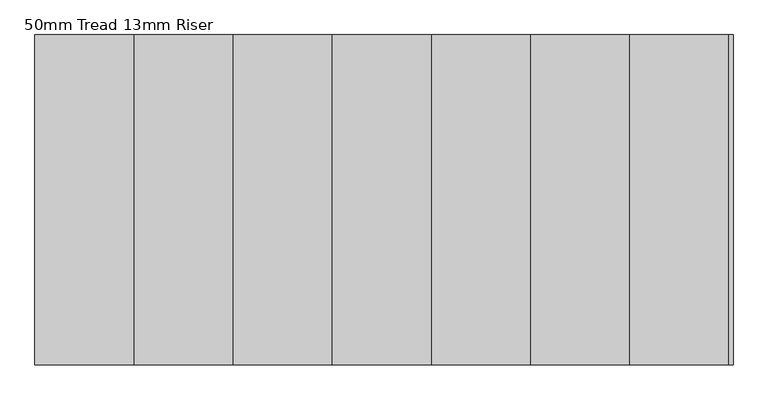
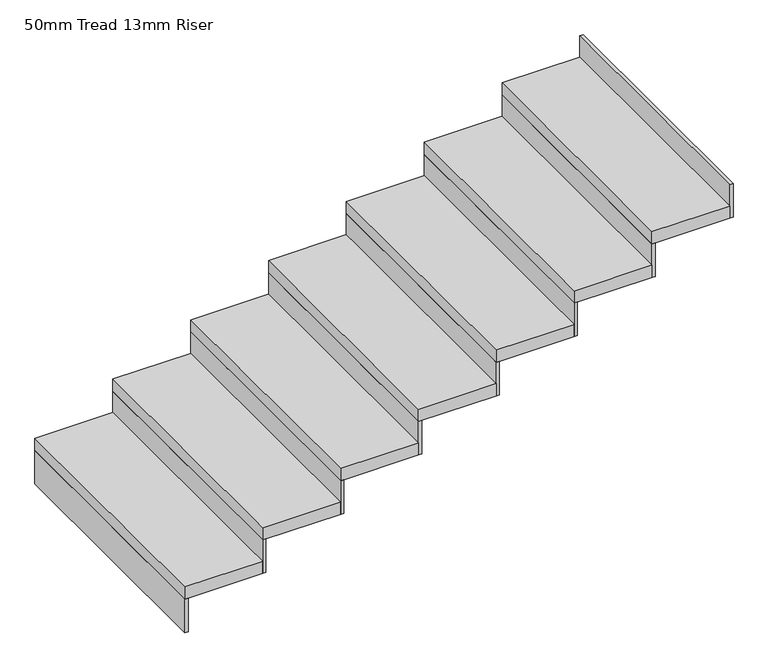
"""IFC4 building model written with IfcOpenShell, lengths in millimetres: stair flight geometry, 50mm Tread 13mm Riser."""

from ifc_helpers import new_model, si_unit, frame, origin, place, context, project, spatial, polyline, outline, extrude, source, transform, mapped, element, save


def stair_flight_50mm_tread_13mm_riser_37edc78a(model_context):
    return source(origin(), model_context, "Body", "SweptSolid", [
        extrude(outline(polyline([(-11937.8449834, -3240.1378151), (-11950.3449834, -3240.1378151), (-11950.3449834, -2240.1378151), (-11937.8449834, -2240.1378151), (-11937.8449834, -3240.1378151)])), frame((0.0, 0.0, 1859.0909091), z_axis=(0.0, 0.0, 1.0), x_axis=(1.0, 0.0, 0.0)), (0.0, 0.0, 1.0), 136.3636364),
        extrude(outline(polyline([(-11650.3449834, -2240.1378151), (-11650.3449834, -3240.1378151), (-11950.3449834, -3240.1378151), (-11950.3449834, -2240.1378151), (-11650.3449834, -2240.1378151)])), frame((0.0, 0.0, 1995.4545455), z_axis=(0.0, 0.0, 1.0), x_axis=(1.0, 0.0, 0.0)), (0.0, 0.0, 1.0), 50.0),
        extrude(outline(polyline([(-11637.8449834, -3240.1378151), (-11650.3449834, -3240.1378151), (-11650.3449834, -2240.1378151), (-11637.8449834, -2240.1378151), (-11637.8449834, -3240.1378151)])), frame((0.0, 0.0, 1995.4545455), z_axis=(0.0, 0.0, 1.0), x_axis=(1.0, 0.0, 0.0)), (0.0, 0.0, 1.0), 136.3636364),
        extrude(outline(polyline([(-11350.3449834, -2240.1378151), (-11350.3449834, -3240.1378151), (-11650.3449834, -3240.1378151), (-11650.3449834, -2240.1378151), (-11350.3449834, -2240.1378151)])), frame((0.0, 0.0, 2131.8181818), z_axis=(0.0, 0.0, 1.0), x_axis=(1.0, 0.0, 0.0)), (0.0, 0.0, 1.0), 50.0),
        extrude(outline(polyline([(-11337.8449834, -3240.1378151), (-11350.3449834, -3240.1378151), (-11350.3449834, -2240.1378151), (-11337.8449834, -2240.1378151), (-11337.8449834, -3240.1378151)])), frame((0.0, 0.0, 2131.8181818), z_axis=(0.0, 0.0, 1.0), x_axis=(1.0, 0.0, 0.0)), (0.0, 0.0, 1.0), 136.3636364),
        extrude(outline(polyline([(-11050.3449834, -2240.1378151), (-11050.3449834, -3240.1378151), (-11350.3449834, -3240.1378151), (-11350.3449834, -2240.1378151), (-11050.3449834, -2240.1378151)])), frame((0.0, 0.0, 2268.1818182), z_axis=(0.0, 0.0, 1.0), x_axis=(1.0, 0.0, 0.0)), (0.0, 0.0, 1.0), 50.0),
        extrude(outline(polyline([(-11037.8449834, -3240.1378151), (-11050.3449834, -3240.1378151), (-11050.3449834, -2240.1378151), (-11037.8449834, -2240.1378151), (-11037.8449834, -3240.1378151)])), frame((0.0, 0.0, 2268.1818182), z_axis=(0.0, 0.0, 1.0), x_axis=(1.0, 0.0, 0.0)), (0.0, 0.0, 1.0), 136.3636364),
        extrude(outline(polyline([(-10750.3449834, -2240.1378151), (-10750.3449834, -3240.1378151), (-11050.3449834, -3240.1378151), (-11050.3449834, -2240.1378151), (-10750.3449834, -2240.1378151)])), frame((0.0, 0.0, 2404.5454545), z_axis=(0.0, 0.0, 1.0), x_axis=(1.0, 0.0, 0.0)), (0.0, 0.0, 1.0), 50.0),
        extrude(outline(polyline([(-10737.8449834, -3240.1378151), (-10750.3449834, -3240.1378151), (-10750.3449834, -2240.1378151), (-10737.8449834, -2240.1378151), (-10737.8449834, -3240.1378151)])), frame((0.0, 0.0, 2404.5454545), z_axis=(0.0, 0.0, 1.0), x_axis=(1.0, 0.0, 0.0)), (0.0, 0.0, 1.0), 136.3636364),
        extrude(outline(polyline([(-10450.3449834, -2240.1378151), (-10450.3449834, -3240.1378151), (-10750.3449834, -3240.1378151), (-10750.3449834, -2240.1378151), (-10450.3449834, -2240.1378151)])), frame((0.0, 0.0, 2540.9090909), z_axis=(0.0, 0.0, 1.0), x_axis=(1.0, 0.0, 0.0)), (0.0, 0.0, 1.0), 50.0),
        extrude(outline(polyline([(-10437.8449834, -3240.1378151), (-10450.3449834, -3240.1378151), (-10450.3449834, -2240.1378151), (-10437.8449834, -2240.1378151), (-10437.8449834, -3240.1378151)])), frame((0.0, 0.0, 2540.9090909), z_axis=(0.0, 0.0, 1.0), x_axis=(1.0, 0.0, 0.0)), (0.0, 0.0, 1.0), 136.3636364),
        extrude(outline(polyline([(-10150.3449834, -2240.1378151), (-10150.3449834, -3240.1378151), (-10450.3449834, -3240.1378151), (-10450.3449834, -2240.1378151), (-10150.3449834, -2240.1378151)])), frame((0.0, 0.0, 2677.2727273), z_axis=(0.0, 0.0, 1.0), x_axis=(1.0, 0.0, 0.0)), (0.0, 0.0, 1.0), 50.0),
        extrude(outline(polyline([(-10137.8449834, -3240.1378151), (-10150.3449834, -3240.1378151), (-10150.3449834, -2240.1378151), (-10137.8449834, -2240.1378151), (-10137.8449834, -3240.1378151)])), frame((0.0, 0.0, 2677.2727273), z_axis=(0.0, 0.0, 1.0), x_axis=(1.0, 0.0, 0.0)), (0.0, 0.0, 1.0), 136.3636364),
        extrude(outline(polyline([(-9850.3449834, -2240.1378151), (-9850.3449834, -3240.1378151), (-10150.3449834, -3240.1378151), (-10150.3449834, -2240.1378151), (-9850.3449834, -2240.1378151)])), frame((0.0, 0.0, 2813.6363636), z_axis=(0.0, 0.0, 1.0), x_axis=(1.0, 0.0, 0.0)), (0.0, 0.0, 1.0), 50.0),
        extrude(outline(polyline([(-9837.8449834, -3240.1378151), (-9850.3449834, -3240.1378151), (-9850.3449834, -2240.1378151), (-9837.8449834, -2240.1378151), (-9837.8449834, -3240.1378151)])), frame((0.0, 0.0, 2813.6363636), z_axis=(0.0, 0.0, 1.0), x_axis=(1.0, 0.0, 0.0)), (0.0, 0.0, 1.0), 136.3636364),
    ])


if __name__ == "__main__":
    model = new_model("IFC4")
    model_context = context("Model", 3, world=origin())
    ifc_project = project(units=[si_unit("LENGTHUNIT", "METRE", prefix="MILLI")], contexts=[model_context])
    site = spatial("IfcSite", under=ifc_project)
    building = spatial("IfcBuilding", under=site)
    placement = place(None, origin())
    stair_flight_50mm_tread_13mm_riser_shape = stair_flight_50mm_tread_13mm_riser_37edc78a(model_context)
    element("IfcStairFlight", 1, ObjectType="50mm Tread 13mm Riser", at=placement, inside=building, context=model_context, shape_type="MappedRepresentation", body=[
        mapped(stair_flight_50mm_tread_13mm_riser_shape, transform((0.0, 0.0, 0.0), x_axis=(1.0, 0.0, 0.0), y_axis=(0.0, 1.0, 0.0), z_axis=(0.0, 0.0, 1.0))),
    ])
    save(model, "model.ifc")
